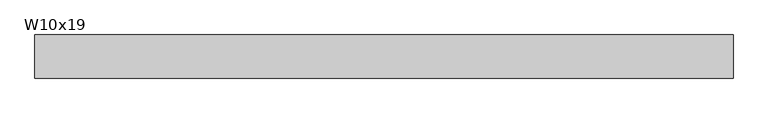
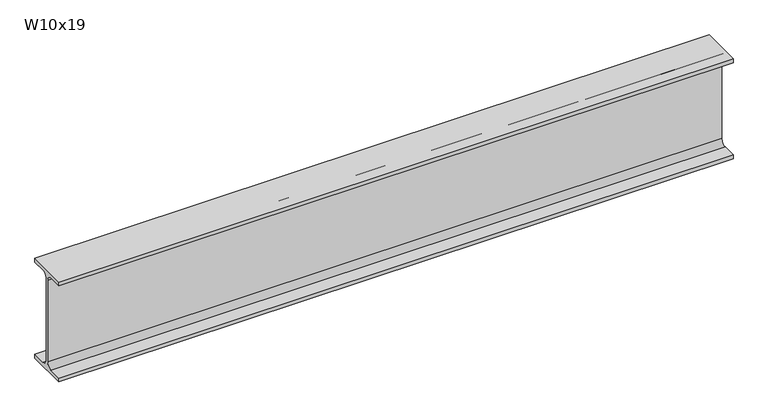
"""IFC4 building model written with IfcOpenShell, lengths in millimetres: beam geometry, RME W-Wide Flange : W10x19."""

from ifc_helpers import new_model, si_unit, point, frame, frame_2d, origin, place, context, project, spatial, polyline, circle_curve, trimmed, segment, composite_curve, outline, extrude, source, transform, mapped, element, save


def w10x19_6eba244d(model_context):
    return source(origin(), model_context, "Body", "SweptSolid", [
        extrude(outline(composite_curve([segment(polyline([(51.054, -119.507), (51.054, -129.54), (-51.054, -129.54), (-51.054, -119.507), (-16.9545, -119.507)]), True, "CONTINUOUS"), segment(trimmed(circle_curve(frame_2d((-16.9545, -105.7275)), 13.7795), [point((-16.9545, -119.507))], [point((-3.175, -105.7275))], True, "CARTESIAN"), True, "CONTINUOUS"), segment(polyline([(-3.175, -105.7275), (-3.175, 105.7275)]), True, "CONTINUOUS"), segment(trimmed(circle_curve(frame_2d((-16.9545, 105.7275)), 13.7795), [point((-3.175, 105.7275))], [point((-16.9545, 119.507))], True, "CARTESIAN"), True, "CONTINUOUS"), segment(polyline([(-16.9545, 119.507), (-51.054, 119.507), (-51.054, 129.54), (51.054, 129.54), (51.054, 119.507), (16.9545, 119.507)]), True, "CONTINUOUS"), segment(trimmed(circle_curve(frame_2d((16.9545, 105.7275)), 13.7795), [point((16.9545, 119.507))], [point((3.175, 105.7275))], True, "CARTESIAN"), True, "CONTINUOUS"), segment(polyline([(3.175, 105.7275), (3.175, -105.7275)]), True, "CONTINUOUS"), segment(trimmed(circle_curve(frame_2d((16.9545, -105.7275)), 13.7795), [point((3.175, -105.7275))], [point((16.9545, -119.507))], True, "CARTESIAN"), True, "CONTINUOUS"), segment(polyline([(16.9545, -119.507), (51.054, -119.507)]), True, "CONTINUOUS")], self_intersect=False)), frame((-826.7881711, 0.0, 0.0), z_axis=(1.0, 0.0, 0.0), x_axis=(0.0, 1.0, 0.0)), (0.0, 0.0, 1.0), 1653.5763422),
    ])


if __name__ == "__main__":
    model = new_model("IFC4")
    model_context = context("Model", 3, world=origin())
    ifc_project = project(units=[si_unit("LENGTHUNIT", "METRE", prefix="MILLI")], contexts=[model_context])
    site = spatial("IfcSite", under=ifc_project)
    building = spatial("IfcBuilding", under=site)
    placement = place(None, origin())
    w10x19_shape = w10x19_6eba244d(model_context)
    element("IfcBeam", 1, ObjectType="RME W-Wide Flange : W10x19", at=placement, inside=building, context=model_context, shape_type="MappedRepresentation", body=[
        mapped(w10x19_shape, transform((0.0, 0.0, 0.0), x_axis=(1.0, 0.0, 0.0), y_axis=(0.0, 1.0, 0.0), z_axis=(0.0, 0.0, 1.0))),
    ])
    save(model, "model.ifc")

# Revit data of these elements
# Type "RME W-Wide Flange : W10x19"
#   WELD P [instance default] = ""
#   WELD LE [instance default] = ""
#   WELD D [instance default] = ""
#   TOP SECTION SIZE [instance default] = ""
#   TOP SECTION LENGTH [instance default] = ""
#   REMARKS [instance default] = ""
#   REINF TYPE [instance default] = ""
#   Nominal Size = "W24"
#   End Bearing Capacity [instance default] = ""
#   BOT SECTION SIZE [instance default] = ""
#   BOT SECTION LENGTH [instance default] = ""
#   Assembly Code = "B10"
#   W = 19
#   Start Extension Calculation [instance default] = 10' - 0"
#   Start Extension [instance default] = -0' - 0 1/2"
#   End Extension Calculation [instance default] = 10' - 0"
#   End Extension [instance default] = -0' - 0 1/2"
#   Length [instance default] = 5' - 0"
#   bf = 0' - 4.02"
#   d = 0' - 10.2"
#   k = 0' - 0 15/16"
#   k2 = 0' - 0.5425"
#   tf = 0' - 0.395"
#   tw = 0' - 0 1/4"
#   A = 0.0390278 SF
#   Structural Material [instance default] = Metal - Steel - ASTM A992
# Element 1 (IfcBeam, "RME W-Wide Flange : W10x19")
#   Length = 5' - 5.10143"
#   Materials on its faces: "Metal - Steel - ASTM A992"
# Materials
#   "Metal - Steel - ASTM A992": class "Metal", colour RGB 255 128 0, transparency 0
